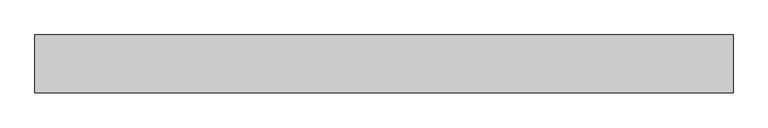
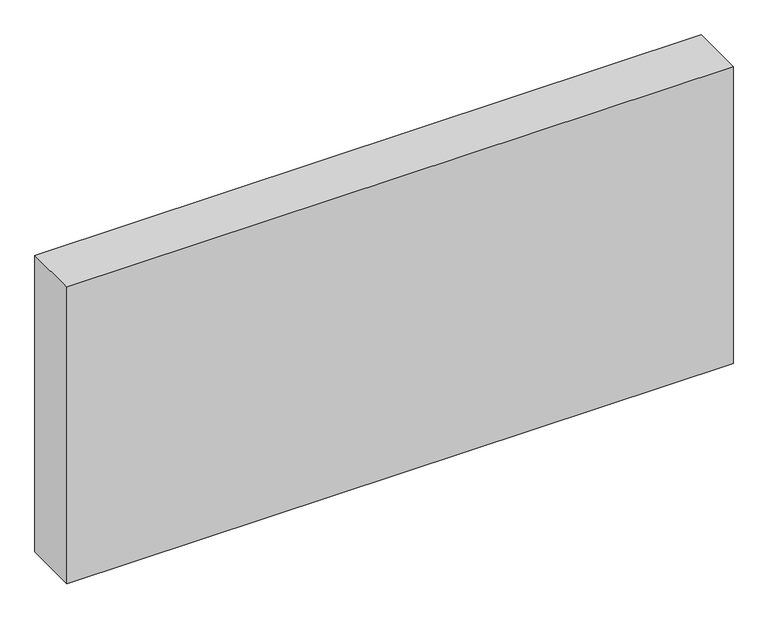
"""IFC4 building model written with IfcOpenShell, lengths in millimetres: proxy geometry, Generic Models 7:Generic Models 1:5:Generic Models 1:5 : Generic Models 7:Generic Models 1:337419:19 : Generic Models 7:Generic Models 1:5:Generic Models 1:5 : Generic Models 7:Generic Models 1:337419:311462."""

from ifc_helpers import new_model, si_unit, frame, origin, place, context, project, spatial, polyline, outline, extrude, source, transform, mapped, element, save


def generic_models_52d90d8b(model_context):
    return source(origin(), model_context, "Body", "SweptSolid", [
        extrude(outline(polyline([(596182.8367239, -578799.0788841), (596182.8367239, -578999.1038841), (593776.1867239, -578999.1038841), (593776.1867239, -578799.0788841), (596182.8367239, -578799.0788841)])), frame((0.0, 0.0, 1311.0765625), z_axis=(0.0, 0.0, 1.0), x_axis=(1.0, 0.0, 0.0)), (0.0, 0.0, 1.0), 1133.871875),
    ])


if __name__ == "__main__":
    model = new_model("IFC4")
    model_context = context("Model", 3, world=origin())
    ifc_project = project(units=[si_unit("LENGTHUNIT", "METRE", prefix="MILLI")], contexts=[model_context])
    site = spatial("IfcSite", under=ifc_project)
    building = spatial("IfcBuilding", under=site)
    placement = place(None, origin())
    generic_models_shape = generic_models_52d90d8b(model_context)
    element("IfcBuildingElementProxy", 1, Name="Generic Models 7:Generic Models 1:5:Generic Models 1:5 : Generic Models 7:Generic Models 1:337419:19 : Generic Models 7:Generic Models 1:5:Generic Models 1:5 : Generic Models 7:Generic Models 1:337419:311462", ObjectType="Generic Models 7:Generic Models 1:5:Generic Models 1:5 : Generic Models 7:Generic Models 1:337419:19 : Generic Models 7:Generic Models 1:5:Generic Models 1:5 : Generic Models 7:Generic Models 1:337419:311462", at=placement, inside=building, context=model_context, shape_type="MappedRepresentation", body=[
        mapped(generic_models_shape, transform((0.0, 0.0, 0.0), x_axis=(1.0, 0.0, 0.0), y_axis=(0.0, 1.0, 0.0), z_axis=(0.0, 0.0, 1.0))),
    ])
    save(model, "model.ifc")

# Revit data of these elements
# Type "Generic Models 7:Generic Models 1:5:Generic Models 1:5 : Generic Models 7:Generic Models 1:337419:19 : Generic Models 7:Generic Models 1:5:Generic Models 1:5 : Generic Models 7:Generic Models 1:337419:311462"
#   NameOverride = "Generic Models 7:Generic Models 1:5:Generic Models 1:5 : Generic Models 7:Generic Models 1:337419:311462"
#   ObjectTypeOverride = "Generic Models 1:5 : Generic Models 7:Generic Models 1:337419"
#   Reference = "Generic Models 1"
#   Tag = "311462"
# Element 1 (IfcBuildingElementProxy, "Generic Models 7:Generic Models 1:5:Generic Models 1:5 : Generic Models 7:Generic Models 1:337419:19 : Generic Models 7:Generic Models 1:5:Generic Models 1:5 : Generic Models 7:Generic Models 1:337419:311462")
#   Materials on its faces: "SIMPLE SAVER INSULATION WITH LINER - COLOR: BLACK"
# Materials
#   "SIMPLE SAVER INSULATION WITH LINER - COLOR: BLACK": class "Unassigned", colour RGB 158 92 175, transparency 0, Cost = 0
